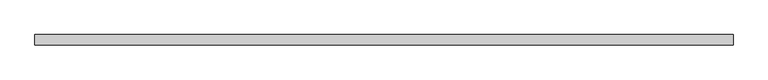
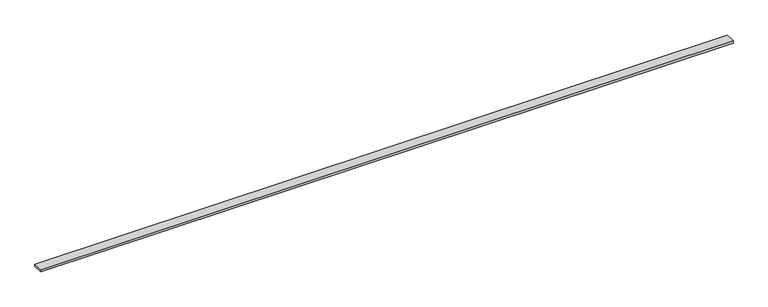
"""IFC4 building model written with IfcOpenShell, lengths in millimetres: proxy geometry, Generic Models 7:Generic Models 1:337419:Generic Models 1:337419 : Generic Models 7:Generic Models 1:337419:34 : Generic Models 7:Generic Models 1:337419:Generic Models 1:337419 : Generic Models 7:Generic Models 1:337419:301336."""

from ifc_helpers import new_model, si_unit, frame, origin, place, context, project, spatial, polyline, outline, extrude, source, transform, mapped, element, save


def generic_models_cdde39f6(model_context):
    return source(origin(), model_context, "Body", "SweptSolid", [
        extrude(outline(polyline([(-578981.6413841, 6128.940625), (-578981.6413841, 6174.978125), (-578797.4913841, 6165.3272324), (-578797.4913841, 6128.940625), (-578981.6413841, 6128.940625)])), frame((560419.6367239, 0.0, 0.0), z_axis=(1.0, 0.0, 0.0), x_axis=(0.0, 1.0, 0.0)), (0.0, 0.0, 1.0), 12477.75),
    ])


if __name__ == "__main__":
    model = new_model("IFC4")
    model_context = context("Model", 3, world=origin())
    ifc_project = project(units=[si_unit("LENGTHUNIT", "METRE", prefix="MILLI")], contexts=[model_context])
    site = spatial("IfcSite", under=ifc_project)
    building = spatial("IfcBuilding", under=site)
    placement = place(None, origin())
    generic_models_shape = generic_models_cdde39f6(model_context)
    element("IfcBuildingElementProxy", 1, Name="Generic Models 7:Generic Models 1:337419:Generic Models 1:337419 : Generic Models 7:Generic Models 1:337419:34 : Generic Models 7:Generic Models 1:337419:Generic Models 1:337419 : Generic Models 7:Generic Models 1:337419:301336", ObjectType="Generic Models 7:Generic Models 1:337419:Generic Models 1:337419 : Generic Models 7:Generic Models 1:337419:34 : Generic Models 7:Generic Models 1:337419:Generic Models 1:337419 : Generic Models 7:Generic Models 1:337419:301336", at=placement, inside=building, context=model_context, shape_type="MappedRepresentation", body=[
        mapped(generic_models_shape, transform((0.0, 0.0, 0.0), x_axis=(1.0, 0.0, 0.0), y_axis=(0.0, 1.0, 0.0), z_axis=(0.0, 0.0, 1.0))),
    ])
    save(model, "model.ifc")

# Revit data of these elements
# Type "Generic Models 7:Generic Models 1:337419:Generic Models 1:337419 : Generic Models 7:Generic Models 1:337419:34 : Generic Models 7:Generic Models 1:337419:Generic Models 1:337419 : Generic Models 7:Generic Models 1:337419:301336"
#   NameOverride = "Generic Models 7:Generic Models 1:337419:Generic Models 1:337419 : Generic Models 7:Generic Models 1:337419:301336"
#   ObjectTypeOverride = "Generic Models 1:337419 : Generic Models 7:Generic Models 1:337419"
#   Reference = "Generic Models 1"
#   Tag = "301336"
# Element 1 (IfcBuildingElementProxy, "Generic Models 7:Generic Models 1:337419:Generic Models 1:337419 : Generic Models 7:Generic Models 1:337419:34 : Generic Models 7:Generic Models 1:337419:Generic Models 1:337419 : Generic Models 7:Generic Models 1:337419:301336")
#   Materials on its faces: "FIRE RETARDTANT WOOD BLOCKING - SIZE AS NECESSARY"
# Materials
#   "FIRE RETARDTANT WOOD BLOCKING - SIZE AS NECESSARY": class "Wood", colour RGB 144 113 62, transparency 0, Description = "Pinus Echinata", Cost = 0
